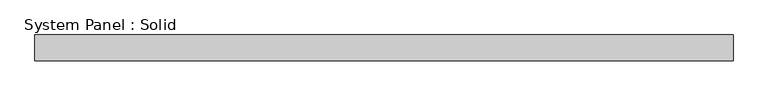
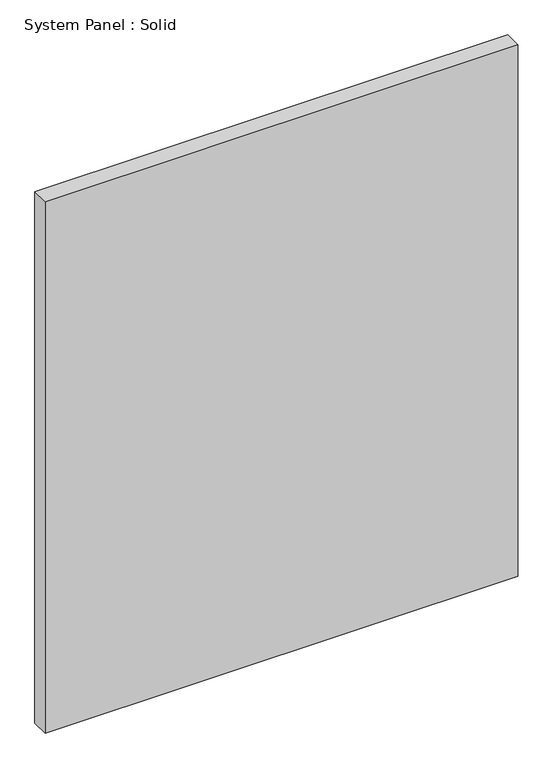
"""IFC4 building model written with IfcOpenShell, lengths in millimetres: plate geometry, System Panel : Solid."""

import ifcopenshell
import ifcopenshell.guid

model = None  # the IFC model being written
_history = None  # IfcOwnerHistory: only IFC2X3 demands one
_inside = {}  # id of a spatial element -> (the spatial element, [elements in it])
_under = {}  # id of a project, library or spatial element -> (it, [spatial elements below it])
_declared = {}  # id of a project -> (the project, [libraries it declares])
_typed = {}  # id of a type object -> (the type object, [elements of that type])
_made_of = {}  # id of a material, layer set ... -> (it, [elements and type objects made of it])


def new_model(schema):
    """Start an empty IFC model of exactly this schema.

    Asked for "IFC4X3", IfcOpenShell would pick the latest addendum, in which some entities
    have other attributes; the version numbers below select the first issue.
    IFC2X3 requires an IfcOwnerHistory on every rooted entity: one is made here for all.
    """
    global model, _history
    if schema == "IFC4X3":
        model = ifcopenshell.file(schema_version=(4, 3, 0, 0))
    else:
        model = ifcopenshell.file(schema=schema)
    _inside.clear()
    _under.clear()
    _declared.clear()
    _typed.clear()
    _made_of.clear()
    _history = None
    if model.schema == "IFC2X3":
        org = make("IfcOrganization", Name="unknown")
        user = make(
            "IfcPersonAndOrganization",
            ThePerson=make("IfcPerson", FamilyName="unknown"),
            TheOrganization=org,
        )
        app = make(
            "IfcApplication",
            ApplicationDeveloper=org,
            Version="unknown",
            ApplicationFullName="unknown",
            ApplicationIdentifier="unknown",
        )
        _history = make(
            "IfcOwnerHistory",
            OwningUser=user,
            OwningApplication=app,
            ChangeAction="ADDED",
            CreationDate=0,
        )
    return model


def make(cls, **values):
    """One entity of the class cls with the attributes given. An attribute that is None is left unset."""
    return model.create_entity(
        cls, **{name: value for name, value in values.items() if value is not None}
    )


def rooted(cls, **values):
    """An entity with a GlobalId (a new one), such as an element, a storey or a relation."""
    return make(cls, GlobalId=ifcopenshell.guid.new(), OwnerHistory=_history, **values)


def si_unit(unit_type, name, prefix=None):
    """IfcSIUnit, for example si_unit("LENGTHUNIT", "METRE", prefix="MILLI")."""
    return make("IfcSIUnit", UnitType=unit_type, Prefix=prefix, Name=name)


def assignment(units):
    """IfcUnitAssignment: the units of a project."""
    return None if units is None else make("IfcUnitAssignment", Units=units)


def point(xyz):
    """IfcCartesianPoint."""
    return None if xyz is None else make("IfcCartesianPoint", Coordinates=xyz)


def direction(xyz):
    """IfcDirection."""
    return None if xyz is None else make("IfcDirection", DirectionRatios=xyz)


def frame(location, z_axis=None, x_axis=None):
    """IfcAxis2Placement3D, a coordinate frame: its origin and axes. An axis left out is left unset."""
    return make(
        "IfcAxis2Placement3D",
        Location=point(location),
        Axis=direction(z_axis),
        RefDirection=direction(x_axis),
    )


def origin():
    """The frame at (0, 0, 0) with its axes left unset."""
    return frame((0.0, 0.0, 0.0))


def origin_with_axes():
    """The frame at (0, 0, 0) with the z axis (0, 0, 1) and the x axis (1, 0, 0) written out."""
    return frame((0.0, 0.0, 0.0), z_axis=(0.0, 0.0, 1.0), x_axis=(1.0, 0.0, 0.0))


def place(relative_to, where):
    """IfcLocalPlacement: puts the frame where relative to a parent placement (None: the world)."""
    return make(
        "IfcLocalPlacement", PlacementRelTo=relative_to, RelativePlacement=where
    )


def context(
    kind, dimensions, precision=None, world=None, true_north=None, identifier=None
):
    """IfcGeometricRepresentationContext, for example the 3D "Model" context."""
    return make(
        "IfcGeometricRepresentationContext",
        ContextIdentifier=identifier,
        ContextType=kind,
        CoordinateSpaceDimension=dimensions,
        Precision=precision,
        WorldCoordinateSystem=world,
        TrueNorth=true_north,
    )


def project(units=None, contexts=None):
    """IfcProject with its units and contexts."""
    return rooted(
        "IfcProject",
        Name="project",
        RepresentationContexts=contexts,
        UnitsInContext=assignment(units),
    )


def spatial(cls, under=None, at=None, **own):
    """A site, building, storey or space (cls), placed at a placement, below another one or the project."""
    s = rooted(cls, ObjectPlacement=at, **own)
    if under is not None:
        _under.setdefault(under.id(), (under, []))[1].append(s)
    return s


def polyline(points):
    """IfcPolyline through the points."""
    return make("IfcPolyline", Points=[point(p) for p in points])


def outline(outer, holes=None, kind="AREA"):
    """IfcArbitraryClosedProfileDef: a profile drawn as a closed curve; with holes, ...WithVoids."""
    if holes is None:
        return make("IfcArbitraryClosedProfileDef", ProfileType=kind, OuterCurve=outer)
    return make(
        "IfcArbitraryProfileDefWithVoids",
        ProfileType=kind,
        OuterCurve=outer,
        InnerCurves=holes,
    )


def extrude(swept, where, along, depth):
    """IfcExtrudedAreaSolid: the profile swept, set in the frame where, extruded along a direction by depth."""
    return make(
        "IfcExtrudedAreaSolid",
        SweptArea=swept,
        Position=where,
        ExtrudedDirection=direction(along),
        Depth=depth,
    )


def shape(context_of_items, identifier, shape_type, items):
    """IfcShapeRepresentation: the items that make up one representation, for example the "Body"."""
    return make(
        "IfcShapeRepresentation",
        ContextOfItems=context_of_items,
        RepresentationIdentifier=identifier,
        RepresentationType=shape_type,
        Items=items,
    )


def source(mapping_origin, context_of_items, identifier, shape_type, items):
    """IfcRepresentationMap: a shape defined once, which mapped items show again and again."""
    return make(
        "IfcRepresentationMap",
        MappingOrigin=mapping_origin,
        MappedRepresentation=shape(context_of_items, identifier, shape_type, items),
    )


def transform(
    local_origin,
    x_axis=None,
    y_axis=None,
    z_axis=None,
    scale=None,
    scale2=None,
    scale3=None,
    uniform=True,
):
    """IfcCartesianTransformationOperator3D, or its non-uniform kind. x_axis, y_axis, z_axis: its Axis1, 2, 3."""
    if uniform:
        return make(
            "IfcCartesianTransformationOperator3D",
            Axis1=direction(x_axis),
            Axis2=direction(y_axis),
            LocalOrigin=point(local_origin),
            Scale=scale,
            Axis3=direction(z_axis),
        )
    return make(
        "IfcCartesianTransformationOperator3DnonUniform",
        Axis1=direction(x_axis),
        Axis2=direction(y_axis),
        LocalOrigin=point(local_origin),
        Scale=scale,
        Axis3=direction(z_axis),
        Scale2=scale2,
        Scale3=scale3,
    )


def mapped(mapping_source, mapping_target):
    """IfcMappedItem: shows the shape of a source again, moved by a transform."""
    return make(
        "IfcMappedItem", MappingSource=mapping_source, MappingTarget=mapping_target
    )


def made_of(thing, what):
    """Note that an element or type object is made of a material, layer set ...; save() writes the relation."""
    if what is not None:
        _made_of.setdefault(what.id(), (what, []))[1].append(thing)
    return thing


def element(
    cls,
    number,
    at=None,
    inside=None,
    cuts=None,
    type_object=None,
    material=None,
    context=None,
    identifier="Body",
    shape_type=None,
    held_by="IfcProductDefinitionShape",
    body=None,
    shapes=None,
    **own,
):
    """One element of the class cls, such as IfcWall. Its Tag is "e" and its number.

    at: its placement. inside: the storey or other place that contains it. cuts: it is an
    opening in that element (IfcRelVoidsElement). A single representation is given by context,
    identifier, shape_type and body (its items); several are given by shapes. held_by: the class
    of the entity that holds the representations. save() writes the other relations.
    """
    e = rooted(cls, Tag="e%d" % number, ObjectPlacement=at, **own)
    if body is not None:
        shapes = [shape(context, identifier, shape_type, body)]
    if shapes is not None:
        e.Representation = make(held_by, Representations=shapes)
    if inside is not None:
        _inside.setdefault(inside.id(), (inside, []))[1].append(e)
    if cuts is not None:
        rooted(
            "IfcRelVoidsElement", RelatingBuildingElement=cuts, RelatedOpeningElement=e
        )
    if type_object is not None:
        _typed.setdefault(type_object.id(), (type_object, []))[1].append(e)
    return made_of(e, material)


def aggregate(whole, parts):
    """IfcRelAggregates: a whole, such as a stair, and the parts it consists of."""
    return rooted("IfcRelAggregates", RelatingObject=whole, RelatedObjects=parts)


def save(model, path):
    """Write the relations noted so far, then the file.

    IfcRelAggregates (storeys below a building ...), IfcRelContainedInSpatialStructure (elements
    in a storey), IfcRelDefinesByType, IfcRelAssociatesMaterial and IfcRelDeclares: one each for
    every whole, place, type object, material and project.
    """
    for whole, parts in _under.values():
        aggregate(whole, parts)
    for where, things in _inside.values():
        rooted(
            "IfcRelContainedInSpatialStructure",
            RelatedElements=things,
            RelatingStructure=where,
        )
    for kind, things in _typed.values():
        rooted("IfcRelDefinesByType", RelatedObjects=things, RelatingType=kind)
    for what, things in _made_of.values():
        rooted("IfcRelAssociatesMaterial", RelatedObjects=things, RelatingMaterial=what)
    for by, libraries in _declared.values():
        rooted("IfcRelDeclares", RelatingContext=by, RelatedDefinitions=libraries)
    model.write(path)


def system_panel_solid_ede99fb6(model_context):
    return source(origin(), model_context, "Body", "SweptSolid", [
        extrude(outline(polyline([(810.0, -10.5), (-810.0, -10.5), (-810.0, 49.5), (810.0, 49.5), (810.0, -10.5)])), origin_with_axes(), (0.0, 0.0, 1.0), 1925.0),
    ])


if __name__ == "__main__":
    model = new_model("IFC4")
    model_context = context("Model", 3, world=origin())
    ifc_project = project(units=[si_unit("LENGTHUNIT", "METRE", prefix="MILLI")], contexts=[model_context])
    site = spatial("IfcSite", under=ifc_project)
    building = spatial("IfcBuilding", under=site)
    placement = place(None, origin())
    system_panel_solid_shape = system_panel_solid_ede99fb6(model_context)
    element("IfcPlate", 1, ObjectType="System Panel : Solid", at=placement, inside=building, context=model_context, shape_type="MappedRepresentation", body=[
        mapped(system_panel_solid_shape, transform((0.0, 0.0, 0.0), x_axis=(1.0, 0.0, 0.0), y_axis=(0.0, 1.0, 0.0), z_axis=(0.0, 0.0, 1.0))),
    ])
    save(model, "model.ifc")

# Revit data of these elements
# Element 1 (IfcPlate, "System Panel : Solid")
#   Materials on its faces: "Default"
# Materials
#   "Default": class "Miscellaneous", colour RGB 127 127 127, transparency 0
